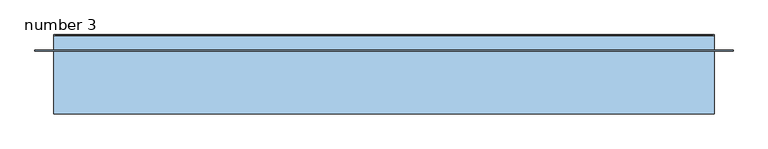
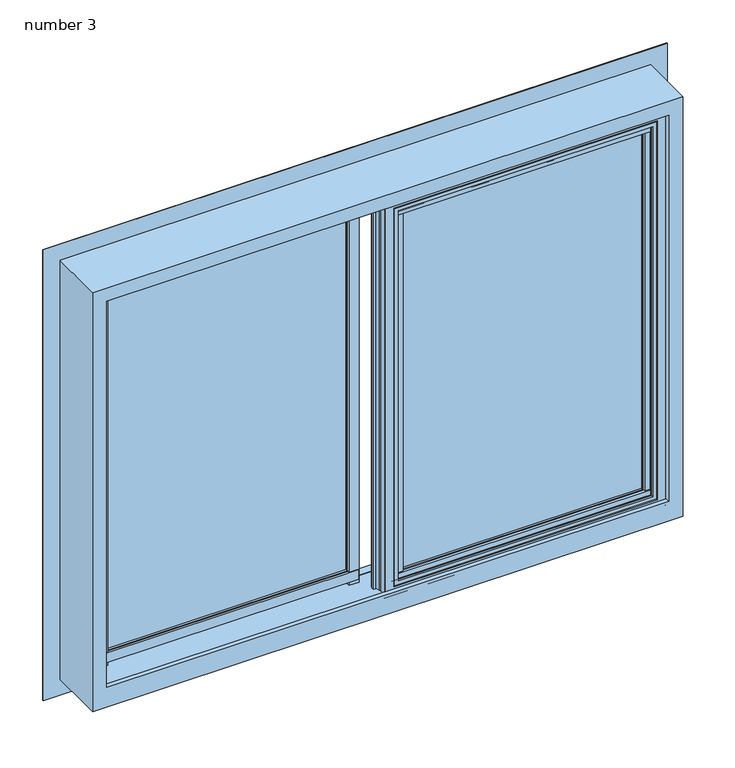
"""IFC4 building model written with IfcOpenShell, lengths in millimetres: window geometry, Window-Exterior-Sierra-Horizontal_Sliding_XO-36inch_Width-Standard : number 3."""

from ifc_helpers import new_model, si_unit, point, frame, frame_2d, origin, place, context, project, spatial, polyline, circle_curve, ellipse_curve, trimmed, segment, composite_curve, outline, extrude, faceted_brep, source, transform, mapped, element, save
from ifc_brep_helpers import plane_surface, cylinder_surface, revolved_surface, advanced_brep


def number_3_fed4ddc9(model_context):
    return source(origin(), model_context, "Body", "SolidModel", [
        extrude(outline(polyline([(-30.95625, 959.3990662), (-42.06875, 960.3157287), (-42.06875, 980.7896808), (-30.95625, 981.7063433), (-30.95625, 959.3990662)])), frame((23.8125, 0.0, 0.0), z_axis=(1.0, 0.0, 0.0), x_axis=(0.0, 1.0, 0.0)), (0.0, 0.0, 1.0), 536.575),
        extrude(outline(polyline([(-11.90625, 981.7063433), (-0.6945312, 980.9337774), (-0.6945312, 960.1716321), (-11.90625, 959.3990662), (-11.90625, 981.7063433)])), frame((23.8125, 0.0, 0.0), z_axis=(1.0, 0.0, 0.0), x_axis=(0.0, 1.0, 0.0)), (0.0, 0.0, 1.0), 536.575),
        extrude(outline(composite_curve([segment(polyline([(-30.95625, 970.5465365), (-30.95625, 959.4453125), (-33.62325, 959.4453125), (-33.62325, 961.0201125)]), True, "CONTINUOUS"), segment(trimmed(circle_curve(frame_2d((-31.4860105, 966.253572)), 5.6530426), [point((-33.62325, 961.0201125))], [point((-37.12845, 966.5996458))], False, "CARTESIAN"), True, "CONTINUOUS"), segment(polyline([(-37.12845, 966.5996458), (-41.275, 966.5996458), (-41.275, 974.5159792), (-39.5097, 974.5159792)]), True, "CONTINUOUS"), segment(trimmed(circle_curve(frame_2d((-31.4860105, 974.862053)), 8.0311494), [point((-39.5097, 974.5159792))], [point((-37.5778298, 980.0955125))], False, "CARTESIAN"), True, "CONTINUOUS"), segment(polyline([(-37.5778298, 980.0955125), (-37.5778298, 981.6703125), (-30.95625, 981.6703125), (-30.95625, 970.5465365)]), True, "CONTINUOUS")], self_intersect=False)), frame((23.8125, 0.0, 0.0), z_axis=(1.0, 0.0, 0.0), x_axis=(0.0, 1.0, 0.0)), (0.0, 0.0, 1.0), 536.575),
        extrude(outline(polyline([(13.890625, 959.3990662), (2.778125, 960.3157287), (2.778125, 980.7896808), (13.890625, 981.7063433), (13.890625, 959.3990662)])), frame((-560.3875, 0.0, 0.0), z_axis=(1.0, 0.0, 0.0), x_axis=(0.0, 1.0, 0.0)), (0.0, 0.0, 1.0), 536.575),
        extrude(outline(polyline([(32.940625, 981.7063433), (44.1523438, 980.9337774), (44.1523438, 960.1716321), (32.940625, 959.3990662), (32.940625, 981.7063433)])), frame((-560.3875, 0.0, 0.0), z_axis=(1.0, 0.0, 0.0), x_axis=(0.0, 1.0, 0.0)), (0.0, 0.0, 1.0), 536.575),
        extrude(outline(composite_curve([segment(polyline([(13.890625, 970.5465365), (13.890625, 959.4453125), (11.223625, 959.4453125), (11.223625, 961.0201125)]), True, "CONTINUOUS"), segment(trimmed(circle_curve(frame_2d((13.3608645, 966.253572)), 5.6530426), [point((11.223625, 961.0201125))], [point((7.718425, 966.5996458))], False, "CARTESIAN"), True, "CONTINUOUS"), segment(polyline([(7.718425, 966.5996458), (3.571875, 966.5996458), (3.571875, 974.5159792), (5.337175, 974.5159792)]), True, "CONTINUOUS"), segment(trimmed(circle_curve(frame_2d((13.3608645, 974.862053)), 8.0311494), [point((5.337175, 974.5159792))], [point((7.2690452, 980.0955125))], False, "CARTESIAN"), True, "CONTINUOUS"), segment(polyline([(7.2690452, 980.0955125), (7.2690452, 981.6703125), (13.890625, 981.6703125), (13.890625, 970.5465365)]), True, "CONTINUOUS")], self_intersect=False)), frame((-560.3875, 0.0, 0.0), z_axis=(1.0, 0.0, 0.0), x_axis=(0.0, 1.0, 0.0)), (0.0, 0.0, 1.0), 536.575),
        extrude(outline(polyline([(13.890625, 1761.4834412), (2.778125, 1762.4001037), (2.778125, 1782.8740558), (13.890625, 1783.7907183), (13.890625, 1761.4834412)])), frame((-560.3875, 0.0, 0.0), z_axis=(1.0, 0.0, 0.0), x_axis=(0.0, 1.0, 0.0)), (0.0, 0.0, 1.0), 536.575),
        extrude(outline(polyline([(32.940625, 1783.7907183), (44.1523438, 1783.0181524), (44.1523438, 1762.2560071), (32.940625, 1761.4834412), (32.940625, 1783.7907183)])), frame((-560.3875, 0.0, 0.0), z_axis=(1.0, 0.0, 0.0), x_axis=(0.0, 1.0, 0.0)), (0.0, 0.0, 1.0), 536.575),
        extrude(outline(composite_curve([segment(polyline([(13.890625, 1772.6309115), (13.890625, 1761.5296875), (11.223625, 1761.5296875), (11.223625, 1763.1044875)]), True, "CONTINUOUS"), segment(trimmed(circle_curve(frame_2d((13.3608645, 1768.337947)), 5.6530426), [point((11.223625, 1763.1044875))], [point((7.718425, 1768.6840208))], False, "CARTESIAN"), True, "CONTINUOUS"), segment(polyline([(7.718425, 1768.6840208), (3.571875, 1768.6840208), (3.571875, 1776.6003542), (5.337175, 1776.6003542)]), True, "CONTINUOUS"), segment(trimmed(circle_curve(frame_2d((13.3608645, 1776.946428)), 8.0311494), [point((5.337175, 1776.6003542))], [point((7.2690452, 1782.1798875))], False, "CARTESIAN"), True, "CONTINUOUS"), segment(polyline([(7.2690452, 1782.1798875), (7.2690452, 1783.7546875), (13.890625, 1783.7546875), (13.890625, 1772.6309115)]), True, "CONTINUOUS")], self_intersect=False)), frame((-560.3875, 0.0, 0.0), z_axis=(1.0, 0.0, 0.0), x_axis=(0.0, 1.0, 0.0)), (0.0, 0.0, 1.0), 536.575),
        extrude(outline(polyline([(-30.95625, 1761.4834412), (-42.06875, 1762.4001037), (-42.06875, 1782.8740558), (-30.95625, 1783.7907183), (-30.95625, 1761.4834412)])), frame((23.8125, 0.0, 0.0), z_axis=(1.0, 0.0, 0.0), x_axis=(0.0, 1.0, 0.0)), (0.0, 0.0, 1.0), 536.575),
        extrude(outline(polyline([(-11.90625, 1783.7907183), (-0.6945312, 1783.0181524), (-0.6945312, 1762.2560071), (-11.90625, 1761.4834412), (-11.90625, 1783.7907183)])), frame((23.8125, 0.0, 0.0), z_axis=(1.0, 0.0, 0.0), x_axis=(0.0, 1.0, 0.0)), (0.0, 0.0, 1.0), 536.575),
        extrude(outline(composite_curve([segment(polyline([(-30.95625, 1772.6309115), (-30.95625, 1761.5296875), (-33.62325, 1761.5296875), (-33.62325, 1763.1044875)]), True, "CONTINUOUS"), segment(trimmed(circle_curve(frame_2d((-31.4860105, 1768.337947)), 5.6530426), [point((-33.62325, 1763.1044875))], [point((-37.12845, 1768.6840208))], False, "CARTESIAN"), True, "CONTINUOUS"), segment(polyline([(-37.12845, 1768.6840208), (-41.275, 1768.6840208), (-41.275, 1776.6003542), (-39.5097, 1776.6003542)]), True, "CONTINUOUS"), segment(trimmed(circle_curve(frame_2d((-31.4860105, 1776.946428)), 8.0311494), [point((-39.5097, 1776.6003542))], [point((-37.5778298, 1782.1798875))], False, "CARTESIAN"), True, "CONTINUOUS"), segment(polyline([(-37.5778298, 1782.1798875), (-37.5778298, 1783.7546875), (-30.95625, 1783.7546875), (-30.95625, 1772.6309115)]), True, "CONTINUOUS")], self_intersect=False)), frame((23.8125, 0.0, 0.0), z_axis=(1.0, 0.0, 0.0), x_axis=(0.0, 1.0, 0.0)), (0.0, 0.0, 1.0), 536.575),
        extrude(outline(polyline([(-563.0134338, 13.890625), (-540.7061567, 13.890625), (-541.6228192, 4.365625), (-562.0967713, 4.365625), (-563.0134338, 13.890625)])), frame((0.0, 0.0, 952.5), z_axis=(0.0, 0.0, 1.0), x_axis=(1.0, 0.0, 0.0)), (0.0, 0.0, 1.0), 838.2),
        extrude(outline(polyline([(-540.7061567, 32.940625), (-563.0134338, 32.940625), (-562.2408679, 42.5648438), (-541.4787226, 42.5648438), (-540.7061567, 32.940625)])), frame((0.0, 0.0, 952.5), z_axis=(0.0, 0.0, 1.0), x_axis=(1.0, 0.0, 0.0)), (0.0, 0.0, 1.0), 838.2),
        extrude(outline(composite_curve([segment(polyline([(-551.8659635, 13.890625), (-540.7421875, 13.890625), (-540.7421875, 9.5985242), (-542.3169875, 9.5985242)]), True, "CONTINUOUS"), segment(trimmed(circle_curve(frame_2d((-547.550447, 13.3608645)), 6.445487), [point((-542.3169875, 9.5985242))], [point((-547.8965208, 6.924675))], False, "CARTESIAN"), True, "CONTINUOUS"), segment(polyline([(-547.8965208, 6.924675), (-547.8965208, 5.159375), (-555.8128542, 5.159375), (-555.8128542, 7.718425)]), True, "CONTINUOUS"), segment(trimmed(circle_curve(frame_2d((-556.158928, 13.3608645)), 5.6530426), [point((-555.8128542, 7.718425))], [point((-561.3923875, 11.223625))], False, "CARTESIAN"), True, "CONTINUOUS"), segment(polyline([(-561.3923875, 11.223625), (-562.9671875, 11.223625), (-562.9671875, 13.890625), (-551.8659635, 13.890625)]), True, "CONTINUOUS")], self_intersect=False)), frame((0.0, 0.0, 952.5), z_axis=(0.0, 0.0, 1.0), x_axis=(1.0, 0.0, 0.0)), (0.0, 0.0, 1.0), 838.2),
        extrude(outline(polyline([(563.0134338, -30.95625), (562.0967713, -40.48125), (541.6228192, -40.48125), (540.7061567, -30.95625), (563.0134338, -30.95625)])), frame((0.0, 0.0, 952.5), z_axis=(0.0, 0.0, 1.0), x_axis=(1.0, 0.0, 0.0)), (0.0, 0.0, 1.0), 838.2),
        extrude(outline(polyline([(540.7061567, -11.90625), (541.4787226, -2.2820312), (562.2408679, -2.2820312), (563.0134338, -11.90625), (540.7061567, -11.90625)])), frame((0.0, 0.0, 952.5), z_axis=(0.0, 0.0, 1.0), x_axis=(1.0, 0.0, 0.0)), (0.0, 0.0, 1.0), 838.2),
        extrude(outline(composite_curve([segment(polyline([(551.8659635, -30.95625), (562.9671875, -30.95625), (562.9671875, -33.62325), (561.3923875, -33.62325)]), True, "CONTINUOUS"), segment(trimmed(circle_curve(frame_2d((556.158928, -31.4860105)), 5.6530426), [point((561.3923875, -33.62325))], [point((555.8128542, -37.12845))], False, "CARTESIAN"), True, "CONTINUOUS"), segment(polyline([(555.8128542, -37.12845), (555.8128542, -39.6875), (547.8965208, -39.6875), (547.8965208, -37.9222)]), True, "CONTINUOUS"), segment(trimmed(circle_curve(frame_2d((547.550447, -31.4860105)), 6.445487), [point((547.8965208, -37.9222))], [point((542.3169875, -35.2483508))], False, "CARTESIAN"), True, "CONTINUOUS"), segment(polyline([(542.3169875, -35.2483508), (540.7421875, -35.2483508), (540.7421875, -30.95625), (551.8659635, -30.95625)]), True, "CONTINUOUS")], self_intersect=False)), frame((0.0, 0.0, 952.5), z_axis=(0.0, 0.0, 1.0), x_axis=(1.0, 0.0, 0.0)), (0.0, 0.0, 1.0), 838.2),
        extrude(outline(polyline([(879.8514818, 644.1495838), (1863.3495838, 644.1495838), (1863.3495838, -644.1495838), (879.8514818, -644.1495838), (879.8514818, 644.1495838)]), holes=[polyline([(914.4200683, -609.5809972), (1828.7809972, -609.5809972), (1828.7809972, 609.5809972), (914.4200683, 609.5809972), (914.4200683, -609.5809972)])]), frame((0.0, 56.35625, 0.0), z_axis=(0.0, 1.0, 0.0), x_axis=(0.0, 0.0, 1.0)), (0.0, 0.0, 1.0), 1.3692925),
        faceted_brep([(592.2452673, 61.8007595, 1811.4452673), (594.5632068, 85.439324, 1813.7632068), (594.5632068, 85.439324, 915.510409), (592.2452673, 61.8007595, 915.510409), (-592.2452673, 61.8007595, 1811.4452673), (-594.5632068, 85.439324, 1813.7632068), (-609.6, -59.8487004, 1828.8), (609.6, -59.8487004, 1828.8), (609.6, 83.8857584, 1828.8), (-609.6, 83.8857584, 1828.8), (-592.2452673, 61.8007595, 915.510409), (-594.5632068, 85.439324, 915.510409), (580.1297286, -59.8487004, 1799.3297286), (580.1297286, -48.9537259, 1799.3297286), (580.1297286, -48.9537259, 950.6555073), (580.1297286, -50.9012589, 951.1326574), (580.1297286, -50.9012589, 957.3267373), (580.1297286, -59.8487004, 957.3267373), (592.6836, -48.9537259, 1811.8836), (592.6836, -1.4525069, 1811.8836), (592.6836, -1.4525069, 939.0175967), (592.6836, -48.9537259, 950.6555073), (583.5400777, -1.4525069, 1802.7400777), (583.5400777, 10.1171482, 1802.7400777), (583.5400777, 10.1171482, 936.1830039), (583.5400777, -1.4525069, 939.0175967), (578.4551976, 10.1171482, 1797.6551976), (578.4551976, 26.899095, 1797.6551976), (578.4551976, 26.899095, 932.0713873), (578.4551976, 10.1171482, 936.1830039), (-609.6, 83.8857584, 915.510409), (-609.6, 86.3576576, 915.510409), (-609.6, 86.3576576, 914.4), (-609.6, -59.8487004, 914.4), (609.6, -59.8487004, 914.4), (609.6, 86.3576576, 914.4), (609.6, 86.3576576, 915.510409), (609.6, 83.8857584, 915.510409), (-580.1297286, -59.8487004, 1799.3297286), (-580.1297286, -59.8487004, 957.3267373), (-580.1297286, -50.9012589, 957.3267373), (-580.1297286, -50.9012589, 951.1326574), (583.6170827, 26.899095, 932.0713873), (583.6170827, 39.894466, 928.8874908), (573.8057011, 41.2733658, 928.5496571), (573.2593437, 52.0255869, 925.9153376), (582.3829219, 52.0255869, 925.9153376), (582.3829219, 55.096925, 925.1628525), (577.977436, 55.096925, 925.1628525), (577.977436, 56.33085, 924.860538), (-577.977436, 56.3169605, 924.8639409), (-577.977436, 55.096925, 925.1628525), (-582.3829219, 55.096925, 925.1628525), (-582.3829219, 52.0255869, 925.9153376), (-573.2593437, 52.0255869, 925.9153376), (-573.8057011, 41.2733658, 928.5496571), (-583.6170827, 39.894466, 928.8874908), (-583.6170827, 26.899095, 932.0713873), (-578.4551976, 26.899095, 932.0713873), (-578.4551976, 10.1171482, 936.1830039), (-583.5400777, 10.1171482, 936.1830039), (-583.5400777, -1.4525069, 939.0175967), (-592.6836, -1.4525069, 939.0175967), (-592.6836, -48.9537259, 950.6555073), (-580.1297286, -48.9537259, 950.6555073), (577.977436, 57.6604904, 924.8639409), (-577.977436, 57.6604904, 924.8639409), (577.977436, 57.6604904, 915.510409), (-577.977436, 57.6604904, 915.510409), (-580.1297286, -48.9537259, 1799.3297286), (-592.6836, -48.9537259, 1811.8836), (-592.6836, -1.4525069, 1811.8836), (-583.5400777, -1.4525069, 1802.7400777), (-583.5400777, 10.1171482, 1802.7400777), (-578.4551976, 10.1171482, 1797.6551976), (-578.4551976, 26.899095, 1797.6551976), (-583.6170827, 26.899095, 1802.8170827), (583.6170827, 26.899095, 1802.8170827), (583.6170827, 39.894466, 1802.8170827), (573.8057011, 41.2733658, 1793.0057011), (-583.6170827, 39.894466, 1802.8170827), (-605.917, 85.439324, 915.510409), (-605.917, 85.439324, 1825.117), (605.917, 85.439324, 1825.117), (605.917, 85.439324, 915.510409), (605.917, 77.5357584, 1825.117), (605.917, 77.5357584, 915.510409), (-605.917, 77.5357584, 1825.117), (-605.917, 77.5357584, 915.510409), (-608.203, 77.5357584, 915.510409), (-608.203, 77.5357584, 1827.403), (608.203, 77.5357584, 1827.403), (608.203, 77.5357584, 915.510409), (608.203, 83.8857584, 1827.403), (608.203, 83.8857584, 915.510409), (-608.203, 83.8857584, 1827.403), (-608.203, 83.8857584, 915.510409), (-584.2071742, 61.8007595, 915.510409), (-584.2071742, 60.6800805, 915.510409), (-577.977436, 60.6800805, 915.510409), (577.977436, 60.6800805, 915.510409), (584.2071742, 60.6800805, 915.510409), (584.2071742, 61.8007595, 915.510409), (-573.8057011, 41.2733658, 1793.0057011), (573.2593437, 52.0255869, 1792.4593437), (-573.2593437, 52.0255869, 1792.4593437), (-582.3829219, 52.0255869, 1801.5829219), (582.3829219, 52.0255869, 1801.5829219), (582.3829219, 55.096925, 1801.5829219), (-582.3829219, 55.096925, 1801.5829219), (-577.977436, 55.096925, 1797.177436), (577.977436, 55.096925, 1797.177436), (577.977436, 60.6800805, 1797.177436), (-577.977436, 60.6800805, 1797.177436), (-584.2071742, 60.6800805, 1803.4071742), (584.2071742, 60.6800805, 1803.4071742), (584.2071742, 61.8007595, 1803.4071742), (-584.2071742, 61.8007595, 1803.4071742)], [[[0, 1, 2, 3]], [[1, 0, 4, 5]], [[6, 7, 8, 9]], [[5, 4, 10, 11]], [[12, 13, 14, 15, 16, 17]], [[18, 19, 20, 21]], [[22, 23, 24, 25]], [[26, 27, 28, 29]], [[6, 9, 30, 31, 32, 33]], [[8, 7, 34, 35, 36, 37]], [[35, 34, 33, 32]], [[7, 6, 33, 34], [38, 12, 17, 39]], [[39, 17, 16, 40]], [[40, 16, 15, 41]], [[41, 15, 14, 21, 20, 25, 24, 29, 28, 42, 43, 44, 45, 46, 47, 48, 49, 50, 51, 52, 53, 54, 55, 56, 57, 58, 59, 60, 61, 62, 63, 64]], [[65, 66, 50, 49]], [[66, 65, 67, 68]], [[13, 69, 64, 63, 70, 18, 21, 14]], [[19, 71, 62, 61, 72, 22, 25, 20]], [[23, 73, 60, 59, 74, 26, 29, 24]], [[27, 75, 58, 57, 76, 77, 42, 28]], [[77, 78, 43, 42]], [[78, 79, 44, 43]], [[12, 38, 69, 13]], [[18, 70, 71, 19]], [[22, 72, 73, 23]], [[26, 74, 75, 27]], [[77, 76, 80, 78]], [[69, 38, 39, 40, 41, 64]], [[71, 70, 63, 62]], [[73, 72, 61, 60]], [[75, 74, 59, 58]], [[80, 76, 57, 56]], [[1, 5, 11, 81, 82, 83, 84, 2]], [[83, 85, 86, 84]], [[85, 87, 88, 89, 90, 91, 92, 86]], [[91, 93, 94, 92]], [[9, 8, 37, 94, 93, 95, 96, 30]], [[83, 82, 87, 85]], [[91, 90, 95, 93]], [[87, 82, 81, 88]], [[95, 90, 89, 96]], [[36, 31, 30, 96, 89, 88, 81, 11, 10, 97, 98, 99, 68, 67, 100, 101, 102, 3, 2, 84, 86, 92, 94, 37]], [[32, 31, 36, 35]], [[79, 78, 80, 103]], [[103, 80, 56, 55]], [[79, 104, 45, 44]], [[104, 105, 54, 53, 106, 107, 46, 45]], [[107, 108, 47, 46]], [[108, 109, 52, 51, 110, 111, 48, 47]], [[111, 112, 100, 67, 65, 49, 48]], [[112, 113, 99, 98, 114, 115, 101, 100]], [[115, 116, 102, 101]], [[4, 0, 3, 102, 116, 117, 97, 10]], [[79, 103, 105, 104]], [[107, 106, 109, 108]], [[111, 110, 113, 112]], [[115, 114, 117, 116]], [[105, 103, 55, 54]], [[109, 106, 53, 52]], [[113, 110, 51, 50, 66, 68, 99]], [[117, 114, 98, 97]]]),
        extrude(outline(polyline([(43.5040588, -30.95625), (42.5873963, -40.48125), (22.1134442, -40.48125), (21.1967817, -30.95625), (43.5040588, -30.95625)])), frame((0.0, 0.0, 952.5), z_axis=(0.0, 0.0, 1.0), x_axis=(1.0, 0.0, 0.0)), (0.0, 0.0, 1.0), 838.2),
        extrude(outline(polyline([(21.1967817, -11.90625), (21.9693476, -2.2820312), (42.7314929, -2.2820312), (43.5040588, -11.90625), (21.1967817, -11.90625)])), frame((0.0, 0.0, 952.5), z_axis=(0.0, 0.0, 1.0), x_axis=(1.0, 0.0, 0.0)), (0.0, 0.0, 1.0), 838.2),
        extrude(outline(composite_curve([segment(polyline([(32.3565885, -30.95625), (43.4578125, -30.95625), (43.4578125, -33.62325), (41.8830125, -33.62325)]), True, "CONTINUOUS"), segment(trimmed(circle_curve(frame_2d((36.649553, -31.4860105)), 5.6530426), [point((41.8830125, -33.62325))], [point((36.3034792, -37.12845))], False, "CARTESIAN"), True, "CONTINUOUS"), segment(polyline([(36.3034792, -37.12845), (36.3034792, -39.6875), (28.3871458, -39.6875), (28.3871458, -37.9222)]), True, "CONTINUOUS"), segment(trimmed(circle_curve(frame_2d((28.041072, -31.4860105)), 6.445487), [point((28.3871458, -37.9222))], [point((22.8076125, -35.2483508))], False, "CARTESIAN"), True, "CONTINUOUS"), segment(polyline([(22.8076125, -35.2483508), (21.2328125, -35.2483508), (21.2328125, -30.95625), (32.3565885, -30.95625)]), True, "CONTINUOUS")], self_intersect=False)), frame((0.0, 0.0, 952.5), z_axis=(0.0, 0.0, 1.0), x_axis=(1.0, 0.0, 0.0)), (0.0, 0.0, 1.0), 838.2),
        extrude(outline(polyline([(-43.5040588, 13.890625), (-21.1967817, 13.890625), (-22.1134442, 4.365625), (-42.5873963, 4.365625), (-43.5040588, 13.890625)])), frame((0.0, 0.0, 952.5), z_axis=(0.0, 0.0, 1.0), x_axis=(1.0, 0.0, 0.0)), (0.0, 0.0, 1.0), 838.2),
        extrude(outline(polyline([(-21.1967817, 32.940625), (-43.5040588, 32.940625), (-42.7314929, 42.5648438), (-21.9693476, 42.5648438), (-21.1967817, 32.940625)])), frame((0.0, 0.0, 952.5), z_axis=(0.0, 0.0, 1.0), x_axis=(1.0, 0.0, 0.0)), (0.0, 0.0, 1.0), 838.2),
        extrude(outline(composite_curve([segment(polyline([(-32.3565885, 13.890625), (-21.2328125, 13.890625), (-21.2328125, 9.5985242), (-22.8076125, 9.5985242)]), True, "CONTINUOUS"), segment(trimmed(circle_curve(frame_2d((-28.041072, 13.3608645)), 6.445487), [point((-22.8076125, 9.5985242))], [point((-28.3871458, 6.924675))], False, "CARTESIAN"), True, "CONTINUOUS"), segment(polyline([(-28.3871458, 6.924675), (-28.3871458, 5.159375), (-36.3034792, 5.159375), (-36.3034792, 7.718425)]), True, "CONTINUOUS"), segment(trimmed(circle_curve(frame_2d((-36.649553, 13.3608645)), 5.6530426), [point((-36.3034792, 7.718425))], [point((-41.8830125, 11.223625))], False, "CARTESIAN"), True, "CONTINUOUS"), segment(polyline([(-41.8830125, 11.223625), (-43.4578125, 11.223625), (-43.4578125, 13.890625), (-32.3565885, 13.890625)]), True, "CONTINUOUS")], self_intersect=False)), frame((0.0, 0.0, 952.5), z_axis=(0.0, 0.0, 1.0), x_axis=(1.0, 0.0, 0.0)), (0.0, 0.0, 1.0), 838.2),
        extrude(outline(polyline([(563.75935, -11.90625), (563.75935, -30.955332), (20.44065, -30.955332), (20.44065, -11.90625), (563.75935, -11.90625)])), frame((0.0, 0.0, 958.65315), z_axis=(0.0, 0.0, 1.0), x_axis=(1.0, 0.0, 0.0)), (0.0, 0.0, 1.0), 825.8937),
        advanced_brep(
        [(554.92015, -9.74725, 967.49235), (29.27985, -9.74725, 967.49235), (29.27985, -10.8831079, 967.49235), (554.92015, -10.8831079, 967.49235), (553.0833265, -7.3042106, 969.3291735), (31.1166735, -7.3042106, 969.3291735), (31.3062238, -9.74725, 969.5187238), (552.8937762, -9.74725, 969.5187238), (560.88915, -4.76885, 961.52335), (23.31085, -4.76885, 961.52335), (560.88915, -2.38125, 961.52335), (23.31085, -2.38125, 961.52335), (585.57795, -4.76885, 936.83455), (-1.37795, -4.76885, 936.83455), (1.00965, -2.38125, 939.22215), (583.19035, -2.38125, 939.22215), (585.57795, -7.33425, 936.83455), (-1.37795, -7.33425, 936.83455), (583.54595, -9.01065, 938.86655), (0.65405, -9.01065, 938.86655), (0.65405, -7.33425, 938.86655), (583.54595, -7.33425, 938.86655), (580.24395, -10.91565, 942.16855), (3.95605, -10.91565, 942.16855), (3.95605, -9.01065, 942.16855), (580.24395, -9.01065, 942.16855), (588.16875, -16.52905, 934.24375), (-3.96875, -16.52905, 934.24375), (-3.96875, -10.91565, 934.24375), (588.16875, -10.91565, 934.24375), (582.86015, -28.72105, 939.55235), (1.33985, -28.72105, 939.55235), (1.33985, -16.52905, 939.55235), (582.86015, -16.52905, 939.55235), (582.86015, -32.68345, 939.55235), (1.33985, -32.68345, 939.55235), (582.86015, -46.01845, 939.55235), (1.33985, -46.01845, 939.55235), (582.04735, -46.83125, 940.36515), (2.15265, -46.83125, 940.36515), (563.75935, -44.950732, 958.65315), (20.44065, -44.950732, 958.65315), (20.44065, -46.83125, 958.65315), (563.75935, -46.83125, 958.65315), (562.1584612, -46.550932, 960.2540388), (22.0415388, -46.550932, 960.2540388), (22.0415388, -44.950732, 960.2540388), (562.1584612, -44.950732, 960.2540388), (554.6146612, -42.7830125, 967.7978388), (29.5853388, -42.7830125, 967.7978388), (29.5853388, -46.550932, 967.7978388), (554.6146612, -46.550932, 967.7978388), (551.4396612, -30.955332, 970.9728388), (32.7603388, -30.955332, 970.9728388), (31.7476888, -42.7830125, 969.9601888), (552.4523112, -42.7830125, 969.9601888), (563.75935, -33.3436209, 958.65315), (20.44065, -33.3436209, 958.65315), (22.8289388, -30.955332, 961.0414388), (561.3710612, -30.955332, 961.0414388), (563.75935, -11.90625, 958.65315), (20.44065, -11.90625, 958.65315), (559.1555891, -10.8831079, 963.2569109), (25.0444109, -10.8831079, 963.2569109), (24.0212688, -11.90625, 962.2337688), (560.1787312, -11.90625, 962.2337688), (29.27985, -9.74725, 1775.70765), (29.27985, -10.8831079, 1775.70765), (31.1166735, -7.3042106, 1773.8708265), (31.3062238, -9.74725, 1773.6812762), (23.31085, -4.76885, 1781.67665), (23.31085, -2.38125, 1781.67665), (-1.37795, -4.76885, 1806.36545), (1.00965, -2.38125, 1803.97785), (-1.37795, -7.33425, 1806.36545), (0.65405, -9.01065, 1804.33345), (0.65405, -7.33425, 1804.33345), (3.95605, -10.91565, 1801.03145), (3.95605, -9.01065, 1801.03145), (-3.96875, -16.52905, 1808.95625), (-3.96875, -10.91565, 1808.95625), (1.33985, -28.72105, 1803.64765), (1.33985, -16.52905, 1803.64765), (1.33985, -32.68345, 1803.64765), (1.33985, -46.01845, 1803.64765), (2.15265, -46.83125, 1802.83485), (20.44065, -44.950732, 1784.54685), (20.44065, -46.83125, 1784.54685), (22.0415388, -46.550932, 1782.9459612), (22.0415388, -44.950732, 1782.9459612), (29.5853388, -42.7830125, 1775.4021612), (29.5853388, -46.550932, 1775.4021612), (32.7603388, -30.955332, 1772.2271612), (31.7476888, -42.7830125, 1773.2398112), (20.44065, -33.3436209, 1784.54685), (22.8289388, -30.955332, 1782.1585612), (20.44065, -11.90625, 1784.54685), (25.0444109, -10.8831079, 1779.9430891), (24.0212688, -11.90625, 1780.9662312), (554.92015, -9.74725, 1775.70765), (554.92015, -10.8831079, 1775.70765), (553.0833265, -7.3042106, 1773.8708265), (552.8937762, -9.74725, 1773.6812762), (560.88915, -4.76885, 1781.67665), (560.88915, -2.38125, 1781.67665), (585.57795, -4.76885, 1806.36545), (583.19035, -2.38125, 1803.97785), (585.57795, -7.33425, 1806.36545), (583.54595, -9.01065, 1804.33345), (583.54595, -7.33425, 1804.33345), (580.24395, -10.91565, 1801.03145), (580.24395, -9.01065, 1801.03145), (588.16875, -16.52905, 1808.95625), (588.16875, -10.91565, 1808.95625), (582.86015, -28.72105, 1803.64765), (582.86015, -16.52905, 1803.64765), (582.86015, -32.68345, 1803.64765), (582.86015, -46.01845, 1803.64765), (582.04735, -46.83125, 1802.83485), (563.75935, -44.950732, 1784.54685), (563.75935, -46.83125, 1784.54685), (562.1584612, -46.550932, 1782.9459612), (562.1584612, -44.950732, 1782.9459612), (554.6146612, -42.7830125, 1775.4021612), (554.6146612, -46.550932, 1775.4021612), (551.4396612, -30.955332, 1772.2271612), (552.4523112, -42.7830125, 1773.2398112), (563.75935, -33.3436209, 1784.54685), (561.3710612, -30.955332, 1782.1585612), (563.75935, -11.90625, 1784.54685), (559.1555891, -10.8831079, 1779.9430891), (560.1787312, -11.90625, 1780.9662312)],
        [
            (0, 1),
            (1, 2),
            (2, 3),
            (3, 0),
            (4, 5),
            (5, 6),
            (6, 7),
            (7, 4),
            (8, 9),
            (9, 5),
            (4, 8),
            (10, 11),
            (11, 9),
            (8, 10),
            (12, 13),
            (13, 14, ellipse_curve(frame((1.00965, -4.76885, 939.22215), z_axis=(0.7071067811865475, 0.0, -0.7071067811865475), x_axis=(0.7071067811865476, 0.0, 0.7071067811865474)), 3.3765763, 2.3876)),
            (14, 15),
            (15, 12, ellipse_curve(frame((583.19035, -4.76885, 939.22215), z_axis=(-0.7071067811865475, 0.0, -0.7071067811865475), x_axis=(0.7071067811865476, 0.0, -0.7071067811865474)), 3.3765763, 2.3876)),
            (16, 17),
            (17, 13),
            (12, 16),
            (18, 19),
            (19, 20),
            (20, 21),
            (21, 18),
            (22, 23),
            (23, 24),
            (24, 25),
            (25, 22),
            (26, 27),
            (27, 28),
            (28, 29),
            (29, 26),
            (30, 31),
            (31, 32),
            (32, 33),
            (33, 30),
            (34, 35),
            (35, 31, ellipse_curve(frame((1.33985, -30.70225, 939.55235), z_axis=(-0.7071067811865475, 0.0, 0.7071067811865475), x_axis=(-0.7071067811865476, 0.0, -0.7071067811865474)), 2.8018399, 1.9812)),
            (30, 34, ellipse_curve(frame((582.86015, -30.70225, 939.55235), z_axis=(0.7071067811865475, 0.0, 0.7071067811865475), x_axis=(-0.7071067811865476, 0.0, 0.7071067811865474)), 2.8018399, 1.9812)),
            (36, 37),
            (37, 35),
            (34, 36),
            (38, 39),
            (39, 37, ellipse_curve(frame((2.15265, -46.01845, 940.36515), z_axis=(0.7071067811865475, 0.0, -0.7071067811865475), x_axis=(0.7071067811865476, 0.0, 0.7071067811865474)), 1.1494728, 0.8128)),
            (36, 38, ellipse_curve(frame((582.04735, -46.01845, 940.36515), z_axis=(-0.7071067811865475, 0.0, -0.7071067811865475), x_axis=(0.7071067811865476, 0.0, -0.7071067811865474)), 1.1494728, 0.8128)),
            (40, 41),
            (41, 42),
            (42, 43),
            (43, 40),
            (44, 45),
            (45, 46),
            (46, 47),
            (47, 44),
            (48, 49),
            (49, 50),
            (50, 51),
            (51, 48),
            (52, 53),
            (53, 54),
            (54, 55),
            (55, 52),
            (56, 57),
            (57, 58),
            (58, 59),
            (59, 56),
            (60, 61),
            (61, 57),
            (56, 60),
            (62, 63),
            (63, 64),
            (64, 65),
            (65, 62),
            (1, 66),
            (66, 67),
            (67, 2),
            (5, 68),
            (68, 69),
            (69, 6),
            (9, 70),
            (70, 68),
            (11, 71),
            (71, 70),
            (13, 72),
            (72, 73, ellipse_curve(frame((1.00965, -4.76885, 1803.97785), z_axis=(-0.7071067811865475, 0.0, -0.7071067811865475), x_axis=(0.7071067811865474, 0.0, -0.7071067811865476)), 3.3765763, 2.3876)),
            (73, 14),
            (17, 74),
            (74, 72),
            (19, 75),
            (75, 76),
            (76, 20),
            (23, 77),
            (77, 78),
            (78, 24),
            (27, 79),
            (79, 80),
            (80, 28),
            (31, 81),
            (81, 82),
            (82, 32),
            (35, 83),
            (83, 81, ellipse_curve(frame((1.33985, -30.70225, 1803.64765), z_axis=(0.7071067811865475, 0.0, 0.7071067811865475), x_axis=(-0.7071067811865474, 0.0, 0.7071067811865476)), 2.8018399, 1.9812)),
            (37, 84),
            (84, 83),
            (39, 85),
            (85, 84, ellipse_curve(frame((2.15265, -46.01845, 1802.83485), z_axis=(-0.7071067811865475, 0.0, -0.7071067811865475), x_axis=(0.7071067811865474, 0.0, -0.7071067811865476)), 1.1494728, 0.8128)),
            (41, 86),
            (86, 87),
            (87, 42),
            (45, 88),
            (88, 89),
            (89, 46),
            (49, 90),
            (90, 91),
            (91, 50),
            (53, 92),
            (92, 93),
            (93, 54),
            (57, 94),
            (94, 95),
            (95, 58),
            (61, 96),
            (96, 94),
            (63, 97),
            (97, 98),
            (98, 64),
            (66, 99),
            (99, 100),
            (100, 67),
            (68, 101),
            (101, 102),
            (102, 69),
            (70, 103),
            (103, 101),
            (71, 104),
            (104, 103),
            (72, 105),
            (105, 106, ellipse_curve(frame((583.19035, -4.76885, 1803.97785), z_axis=(-0.7071067811865475, 0.0, 0.7071067811865475), x_axis=(-0.7071067811865476, 0.0, -0.7071067811865474)), 3.3765763, 2.3876)),
            (106, 73),
            (74, 107),
            (107, 105),
            (75, 108),
            (108, 109),
            (109, 76),
            (77, 110),
            (110, 111),
            (111, 78),
            (79, 112),
            (112, 113),
            (113, 80),
            (81, 114),
            (114, 115),
            (115, 82),
            (83, 116),
            (116, 114, ellipse_curve(frame((582.86015, -30.70225, 1803.64765), z_axis=(0.7071067811865475, 0.0, -0.7071067811865475), x_axis=(0.7071067811865476, 0.0, 0.7071067811865474)), 2.8018399, 1.9812)),
            (84, 117),
            (117, 116),
            (85, 118),
            (118, 117, ellipse_curve(frame((582.04735, -46.01845, 1802.83485), z_axis=(-0.7071067811865475, 0.0, 0.7071067811865475), x_axis=(-0.7071067811865476, 0.0, -0.7071067811865474)), 1.1494728, 0.8128)),
            (86, 119),
            (119, 120),
            (120, 87),
            (88, 121),
            (121, 122),
            (122, 89),
            (90, 123),
            (123, 124),
            (124, 91),
            (92, 125),
            (125, 126),
            (126, 93),
            (94, 127),
            (127, 128),
            (128, 95),
            (96, 129),
            (129, 127),
            (97, 130),
            (130, 131),
            (131, 98),
            (62, 130),
            (100, 3),
            (99, 0),
            (102, 7),
            (101, 4),
            (103, 8),
            (104, 10),
            (106, 15),
            (105, 12),
            (107, 16),
            (109, 21),
            (108, 18),
            (111, 25),
            (110, 22),
            (113, 29),
            (112, 26),
            (115, 33),
            (114, 30),
            (116, 34),
            (117, 36),
            (118, 38),
            (120, 43),
            (119, 40),
            (122, 47),
            (121, 44),
            (124, 51),
            (123, 48),
            (126, 55),
            (125, 52),
            (128, 59),
            (127, 56),
            (129, 60),
            (131, 65),
        ],
        [
            plane_surface(frame((554.92015, -10.8831079, 967.49235), z_axis=(0.0, 0.0, 1.0), x_axis=(-1.0, 0.0, 0.0))),
            plane_surface(frame((552.8937762, -9.74725, 969.5187238), z_axis=(0.0, 0.07735544009934271, 0.9970035786731345), x_axis=(-1.0, 0.0, 0.0))),
            plane_surface(frame((553.0833265, -7.3042106, 969.3291735), z_axis=(0.0, 0.9510889261909004, 0.3089172291683326), x_axis=(-1.0, 0.0, 0.0))),
            plane_surface(frame((560.88915, -4.76885, 961.52335), z_axis=(0.0, 0.0, 1.0), x_axis=(-1.0, 0.0, 0.0))),
            cylinder_surface(frame((588.16875, -4.76885, 939.22215), z_axis=(1.0, 0.0, 0.0), x_axis=(0.0, -1.0, 0.0)), 2.3876),
            plane_surface(frame((585.57795, -4.76885, 936.83455), z_axis=(0.0, 0.0, -1.0), x_axis=(-1.0, 0.0, 0.0))),
            plane_surface(frame((583.54595, -7.33425, 938.86655), z_axis=(0.0, 0.0, -1.0), x_axis=(-1.0, 0.0, 0.0))),
            plane_surface(frame((580.24395, -9.01065, 942.16855), z_axis=(0.0, 0.0, -1.0), x_axis=(-1.0, 0.0, 0.0))),
            plane_surface(frame((588.16875, -10.91565, 934.24375), z_axis=(0.0, 0.0, -1.0), x_axis=(-1.0, 0.0, 0.0))),
            plane_surface(frame((582.86015, -16.52905, 939.55235), z_axis=(0.0, 0.0, -1.0), x_axis=(-1.0, 0.0, 0.0))),
            revolved_surface(polyline([(-0.6413499930890794, -32.68345, 939.55235), (584.841349993089, -32.68345, 939.55235)]), (588.16875, -30.70225, 939.55235), (-1.0, 0.0, 0.0)),
            plane_surface(frame((582.86015, -32.68345, 939.55235), z_axis=(0.0, 0.0, -1.0), x_axis=(-1.0, 0.0, 0.0))),
            cylinder_surface(frame((588.16875, -46.01845, 940.36515), z_axis=(1.0, 0.0, 0.0), x_axis=(0.0, -1.0, 0.0)), 0.8128),
            plane_surface(frame((563.75935, -46.83125, 958.65315), z_axis=(0.0, 0.0, 1.0), x_axis=(-1.0, 0.0, 0.0))),
            plane_surface(frame((562.1584612, -44.950732, 960.2540388), z_axis=(0.0, 0.0, -1.0), x_axis=(-1.0, 0.0, 0.0))),
            plane_surface(frame((554.6146612, -46.550932, 967.7978388), z_axis=(0.0, 0.0, 1.0), x_axis=(-1.0, 0.0, 0.0))),
            plane_surface(frame((552.4523112, -42.7830125, 969.9601888), z_axis=(0.0, -0.08530487454184647, 0.996354895797376), x_axis=(-1.0, 0.0, 0.0))),
            plane_surface(frame((561.3710612, -30.955332, 961.0414388), z_axis=(0.0, 0.7071067811865713, -0.7071067811865238), x_axis=(-1.0, 0.0, 0.0))),
            plane_surface(frame((563.75935, -33.3436209, 958.65315), z_axis=(0.0, 0.0, 1.0), x_axis=(-1.0, 0.0, 0.0))),
            plane_surface(frame((560.1787312, -11.90625, 962.2337688), z_axis=(0.0, -0.7071067811861558, 0.7071067811869393), x_axis=(-1.0, 0.0, 0.0))),
            plane_surface(frame((29.27985, -10.8831079, 967.49235), z_axis=(1.0, 0.0, 0.0), x_axis=(0.0, 0.0, 1.0))),
            plane_surface(frame((31.3062238, -9.74725, 969.5187238), z_axis=(0.9970035786731345, 0.07735544009934266, 0.0), x_axis=(0.0, 0.0, 1.0))),
            plane_surface(frame((31.1166735, -7.3042106, 969.3291735), z_axis=(0.30891722916833264, 0.9510889261909004, 0.0), x_axis=(0.0, 0.0, 1.0))),
            plane_surface(frame((23.31085, -4.76885, 961.52335), z_axis=(1.0, 0.0, 0.0), x_axis=(0.0, 0.0, 1.0))),
            cylinder_surface(frame((1.00965, -4.76885, 934.24375), z_axis=(0.0, 0.0, -1.0), x_axis=(0.0, -1.0, 0.0)), 2.3876),
            plane_surface(frame((-1.37795, -4.76885, 936.83455), z_axis=(-1.0, 0.0, 0.0), x_axis=(0.0, 0.0, 1.0))),
            plane_surface(frame((0.65405, -7.33425, 938.86655), z_axis=(-1.0, 0.0, 0.0), x_axis=(0.0, 0.0, 1.0))),
            plane_surface(frame((3.95605, -9.01065, 942.16855), z_axis=(-1.0, 0.0, 0.0), x_axis=(0.0, 0.0, 1.0))),
            plane_surface(frame((-3.96875, -10.91565, 934.24375), z_axis=(-1.0, 0.0, 0.0), x_axis=(0.0, 0.0, 1.0))),
            plane_surface(frame((1.33985, -16.52905, 939.55235), z_axis=(-1.0, 0.0, 0.0), x_axis=(0.0, 0.0, 1.0))),
            revolved_surface(polyline([(1.33985, -32.68345, 1805.6288499930893), (1.33985, -32.68345, 937.571150006911)]), (1.33985, -30.70225, 934.24375), (0.0, 0.0, 1.0)),
            plane_surface(frame((1.33985, -32.68345, 939.55235), z_axis=(-1.0, 0.0, 0.0), x_axis=(0.0, 0.0, 1.0))),
            cylinder_surface(frame((2.15265, -46.01845, 934.24375), z_axis=(0.0, 0.0, -1.0), x_axis=(0.0, -1.0, 0.0)), 0.8128),
            plane_surface(frame((20.44065, -46.83125, 958.65315), z_axis=(1.0, 0.0, 0.0), x_axis=(0.0, 0.0, 1.0))),
            plane_surface(frame((22.0415388, -44.950732, 960.2540388), z_axis=(-1.0, 0.0, 0.0), x_axis=(0.0, 0.0, 1.0))),
            plane_surface(frame((29.5853388, -46.550932, 967.7978388), z_axis=(1.0, 0.0, 0.0), x_axis=(0.0, 0.0, 1.0))),
            plane_surface(frame((31.7476888, -42.7830125, 969.9601888), z_axis=(0.996354895797376, -0.08530487454184653, 0.0), x_axis=(0.0, 0.0, 1.0))),
            plane_surface(frame((22.8289388, -30.955332, 961.0414388), z_axis=(-0.7071067811865238, 0.7071067811865713, 0.0), x_axis=(0.0, 0.0, 1.0))),
            plane_surface(frame((20.44065, -33.3436209, 958.65315), z_axis=(1.0, 0.0, 0.0), x_axis=(0.0, 0.0, 1.0))),
            plane_surface(frame((24.0212688, -11.90625, 962.2337688), z_axis=(0.7071067811869393, -0.7071067811861558, 0.0), x_axis=(0.0, 0.0, 1.0))),
            plane_surface(frame((29.27985, -10.8831079, 1775.70765), z_axis=(0.0, 0.0, -1.0), x_axis=(1.0, 0.0, 0.0))),
            plane_surface(frame((31.3062238, -9.74725, 1773.6812762), z_axis=(0.0, 0.0773554400993426, -0.9970035786731345), x_axis=(1.0, 0.0, 0.0))),
            plane_surface(frame((31.1166735, -7.3042106, 1773.8708265), z_axis=(0.0, 0.9510889261909004, -0.3089172291683327), x_axis=(1.0, 0.0, 0.0))),
            plane_surface(frame((23.31085, -4.76885, 1781.67665), z_axis=(0.0, 0.0, -1.0), x_axis=(1.0, 0.0, 0.0))),
            cylinder_surface(frame((-3.96875, -4.76885, 1803.97785), z_axis=(-1.0, 0.0, 0.0), x_axis=(0.0, -1.0, 0.0)), 2.3876),
            plane_surface(frame((-1.37795, -4.76885, 1806.36545), z_axis=(0.0, 0.0, 1.0), x_axis=(1.0, 0.0, 0.0))),
            plane_surface(frame((0.65405, -7.33425, 1804.33345), z_axis=(0.0, 0.0, 1.0), x_axis=(1.0, 0.0, 0.0))),
            plane_surface(frame((3.95605, -9.01065, 1801.03145), z_axis=(0.0, 0.0, 1.0), x_axis=(1.0, 0.0, 0.0))),
            plane_surface(frame((-3.96875, -10.91565, 1808.95625), z_axis=(0.0, 0.0, 1.0), x_axis=(1.0, 0.0, 0.0))),
            plane_surface(frame((1.33985, -16.52905, 1803.64765), z_axis=(0.0, 0.0, 1.0), x_axis=(1.0, 0.0, 0.0))),
            revolved_surface(polyline([(584.841349993089, -32.68345, 1803.64765), (-0.6413499930890376, -32.68345, 1803.64765)]), (-3.96875, -30.70225, 1803.64765), (1.0, 0.0, 0.0)),
            plane_surface(frame((1.33985, -32.68345, 1803.64765), z_axis=(0.0, 0.0, 1.0), x_axis=(1.0, 0.0, 0.0))),
            cylinder_surface(frame((-3.96875, -46.01845, 1802.83485), z_axis=(-1.0, 0.0, 0.0), x_axis=(0.0, -1.0, 0.0)), 0.8128),
            plane_surface(frame((20.44065, -46.83125, 1784.54685), z_axis=(0.0, 0.0, -1.0), x_axis=(1.0, 0.0, 0.0))),
            plane_surface(frame((22.0415388, -44.950732, 1782.9459612), z_axis=(0.0, 0.0, 1.0), x_axis=(1.0, 0.0, 0.0))),
            plane_surface(frame((29.5853388, -46.550932, 1775.4021612), z_axis=(0.0, 0.0, -1.0), x_axis=(1.0, 0.0, 0.0))),
            plane_surface(frame((31.7476888, -42.7830125, 1773.2398112), z_axis=(0.0, -0.08530487454184658, -0.996354895797376), x_axis=(1.0, 0.0, 0.0))),
            plane_surface(frame((22.8289388, -30.955332, 1782.1585612), z_axis=(0.0, 0.7071067811865713, 0.7071067811865238), x_axis=(1.0, 0.0, 0.0))),
            plane_surface(frame((20.44065, -33.3436209, 1784.54685), z_axis=(0.0, 0.0, -1.0), x_axis=(1.0, 0.0, 0.0))),
            plane_surface(frame((24.0212688, -11.90625, 1780.9662312), z_axis=(0.0, -0.7071067811861558, -0.7071067811869393), x_axis=(1.0, 0.0, 0.0))),
            plane_surface(frame((559.1555891, -10.8831079, 1779.9430891), z_axis=(0.0, -1.0, 0.0), x_axis=(0.0, 0.0, -1.0))),
            plane_surface(frame((554.92015, -10.8831079, 1775.70765), z_axis=(-1.0, 0.0, 0.0), x_axis=(0.0, 0.0, -1.0))),
            plane_surface(frame((554.92015, -9.74725, 1775.70765), z_axis=(0.0, -1.0, 0.0), x_axis=(0.0, 0.0, -1.0))),
            plane_surface(frame((552.8937762, -9.74725, 1773.6812762), z_axis=(-0.9970035786731345, 0.07735544009934266, 0.0), x_axis=(0.0, 0.0, -1.0))),
            plane_surface(frame((553.0833265, -7.3042106, 1773.8708265), z_axis=(-0.30891722916833264, 0.9510889261909004, 0.0), x_axis=(0.0, 0.0, -1.0))),
            plane_surface(frame((560.88915, -4.76885, 1781.67665), z_axis=(-1.0, 0.0, 0.0), x_axis=(0.0, 0.0, -1.0))),
            plane_surface(frame((560.88915, -2.38125, 1781.67665), z_axis=(0.0, 1.0, 0.0), x_axis=(0.0, 0.0, -1.0))),
            cylinder_surface(frame((583.19035, -4.76885, 1808.95625), z_axis=(0.0, 0.0, 1.0), x_axis=(0.0, -1.0, 0.0)), 2.3876),
            plane_surface(frame((585.57795, -4.76885, 1806.36545), z_axis=(1.0, 0.0, 0.0), x_axis=(0.0, 0.0, -1.0))),
            plane_surface(frame((585.57795, -7.33425, 1806.36545), z_axis=(0.0, -1.0, 0.0), x_axis=(0.0, 0.0, -1.0))),
            plane_surface(frame((583.54595, -7.33425, 1804.33345), z_axis=(1.0, 0.0, 0.0), x_axis=(0.0, 0.0, -1.0))),
            plane_surface(frame((583.54595, -9.01065, 1804.33345), z_axis=(0.0, -1.0, 0.0), x_axis=(0.0, 0.0, -1.0))),
            plane_surface(frame((580.24395, -9.01065, 1801.03145), z_axis=(1.0, 0.0, 0.0), x_axis=(0.0, 0.0, -1.0))),
            plane_surface(frame((580.24395, -10.91565, 1801.03145), z_axis=(0.0, 1.0, 0.0), x_axis=(0.0, 0.0, -1.0))),
            plane_surface(frame((588.16875, -10.91565, 1808.95625), z_axis=(1.0, 0.0, 0.0), x_axis=(0.0, 0.0, -1.0))),
            plane_surface(frame((588.16875, -16.52905, 1808.95625), z_axis=(0.0, -1.0, 0.0), x_axis=(0.0, 0.0, -1.0))),
            plane_surface(frame((582.86015, -16.52905, 1803.64765), z_axis=(1.0, 0.0, 0.0), x_axis=(0.0, 0.0, -1.0))),
            revolved_surface(polyline([(582.86015, -32.68345, 937.571150006911), (582.86015, -32.68345, 1805.6288499930893)]), (582.86015, -30.70225, 1808.95625), (0.0, 0.0, -1.0)),
            plane_surface(frame((582.86015, -32.68345, 1803.64765), z_axis=(1.0, 0.0, 0.0), x_axis=(0.0, 0.0, -1.0))),
            cylinder_surface(frame((582.04735, -46.01845, 1808.95625), z_axis=(0.0, 0.0, 1.0), x_axis=(0.0, -1.0, 0.0)), 0.8128),
            plane_surface(frame((582.04735, -46.83125, 1802.83485), z_axis=(0.0, -1.0, 0.0), x_axis=(0.0, 0.0, -1.0))),
            plane_surface(frame((563.75935, -46.83125, 1784.54685), z_axis=(-1.0, 0.0, 0.0), x_axis=(0.0, 0.0, -1.0))),
            plane_surface(frame((563.75935, -44.950732, 1784.54685), z_axis=(0.0, -1.0, 0.0), x_axis=(0.0, 0.0, -1.0))),
            plane_surface(frame((562.1584612, -44.950732, 1782.9459612), z_axis=(1.0, 0.0, 0.0), x_axis=(0.0, 0.0, -1.0))),
            plane_surface(frame((562.1584612, -46.550932, 1782.9459612), z_axis=(0.0, -1.0, 0.0), x_axis=(0.0, 0.0, -1.0))),
            plane_surface(frame((554.6146612, -46.550932, 1775.4021612), z_axis=(-1.0, 0.0, 0.0), x_axis=(0.0, 0.0, -1.0))),
            plane_surface(frame((554.6146612, -42.7830125, 1775.4021612), z_axis=(0.0, -1.0, 0.0), x_axis=(0.0, 0.0, -1.0))),
            plane_surface(frame((552.4523112, -42.7830125, 1773.2398112), z_axis=(-0.996354895797376, -0.08530487454184653, 0.0), x_axis=(0.0, 0.0, -1.0))),
            plane_surface(frame((551.4396612, -30.955332, 1772.2271612), z_axis=(0.0, 1.0, 0.0), x_axis=(0.0, 0.0, -1.0))),
            plane_surface(frame((561.3710612, -30.955332, 1782.1585612), z_axis=(0.7071067811865238, 0.7071067811865713, 0.0), x_axis=(0.0, 0.0, -1.0))),
            plane_surface(frame((563.75935, -33.3436209, 1784.54685), z_axis=(-1.0, 0.0, 0.0), x_axis=(0.0, 0.0, -1.0))),
            plane_surface(frame((563.75935, -11.90625, 1784.54685), z_axis=(0.0, -1.0, 0.0), x_axis=(0.0, 0.0, -1.0))),
            plane_surface(frame((560.1787312, -11.90625, 1780.9662312), z_axis=(-0.7071067811869393, -0.7071067811861558, 0.0), x_axis=(0.0, 0.0, -1.0))),
        ],
        [
            (0, [[1, 2, 3, 4]]),
            (1, [[5, 6, 7, 8]]),
            (2, [[9, 10, -5, 11]]),
            (3, [[12, 13, -9, 14]]),
            (4, [[15, 16, 17, 18]]),
            (5, [[19, 20, -15, 21]]),
            (6, [[22, 23, 24, 25]]),
            (7, [[26, 27, 28, 29]]),
            (8, [[30, 31, 32, 33]]),
            (9, [[34, 35, 36, 37]]),
            (10, [[38, 39, -34, 40]]),
            (11, [[41, 42, -38, 43]]),
            (12, [[44, 45, -41, 46]]),
            (13, [[47, 48, 49, 50]]),
            (14, [[51, 52, 53, 54]]),
            (15, [[55, 56, 57, 58]]),
            (16, [[59, 60, 61, 62]]),
            (17, [[63, 64, 65, 66]]),
            (18, [[67, 68, -63, 69]]),
            (19, [[70, 71, 72, 73]]),
            (20, [[74, 75, 76, -2]]),
            (21, [[77, 78, 79, -6]]),
            (22, [[80, 81, -77, -10]]),
            (23, [[82, 83, -80, -13]]),
            (24, [[84, 85, 86, -16]]),
            (25, [[87, 88, -84, -20]]),
            (26, [[89, 90, 91, -23]]),
            (27, [[92, 93, 94, -27]]),
            (28, [[95, 96, 97, -31]]),
            (29, [[98, 99, 100, -35]]),
            (30, [[101, 102, -98, -39]]),
            (31, [[103, 104, -101, -42]]),
            (32, [[105, 106, -103, -45]]),
            (33, [[107, 108, 109, -48]]),
            (34, [[110, 111, 112, -52]]),
            (35, [[113, 114, 115, -56]]),
            (36, [[116, 117, 118, -60]]),
            (37, [[119, 120, 121, -64]]),
            (38, [[122, 123, -119, -68]]),
            (39, [[124, 125, 126, -71]]),
            (40, [[127, 128, 129, -75]]),
            (41, [[130, 131, 132, -78]]),
            (42, [[133, 134, -130, -81]]),
            (43, [[135, 136, -133, -83]]),
            (44, [[137, 138, 139, -85]]),
            (45, [[140, 141, -137, -88]]),
            (46, [[142, 143, 144, -90]]),
            (47, [[145, 146, 147, -93]]),
            (48, [[148, 149, 150, -96]]),
            (49, [[151, 152, 153, -99]]),
            (50, [[154, 155, -151, -102]]),
            (51, [[156, 157, -154, -104]]),
            (52, [[158, 159, -156, -106]]),
            (53, [[160, 161, 162, -108]]),
            (54, [[163, 164, 165, -111]]),
            (55, [[166, 167, 168, -114]]),
            (56, [[169, 170, 171, -117]]),
            (57, [[172, 173, 174, -120]]),
            (58, [[175, 176, -172, -123]]),
            (59, [[177, 178, 179, -125]]),
            (60, [[-70, 180, -177, -124], [-3, -76, -129, 181]]),
            (61, [[182, -4, -181, -128]]),
            (62, [[-1, -182, -127, -74], [-7, -79, -132, 183]]),
            (63, [[184, -8, -183, -131]]),
            (64, [[185, -11, -184, -134]]),
            (65, [[186, -14, -185, -136]]),
            (66, [[-17, -86, -139, 187], [-12, -186, -135, -82]]),
            (67, [[188, -18, -187, -138]]),
            (68, [[189, -21, -188, -141]]),
            (69, [[-19, -189, -140, -87], [-24, -91, -144, 190]]),
            (70, [[191, -25, -190, -143]]),
            (71, [[-22, -191, -142, -89], [-28, -94, -147, 192]]),
            (72, [[193, -29, -192, -146]]),
            (73, [[-32, -97, -150, 194], [-26, -193, -145, -92]]),
            (74, [[195, -33, -194, -149]]),
            (75, [[-30, -195, -148, -95], [-36, -100, -153, 196]]),
            (76, [[197, -37, -196, -152]]),
            (77, [[198, -40, -197, -155]]),
            (78, [[199, -43, -198, -157]]),
            (79, [[200, -46, -199, -159]]),
            (80, [[-44, -200, -158, -105], [-49, -109, -162, 201]]),
            (81, [[202, -50, -201, -161]]),
            (82, [[-47, -202, -160, -107], [-53, -112, -165, 203]]),
            (83, [[204, -54, -203, -164]]),
            (84, [[-51, -204, -163, -110], [-57, -115, -168, 205]]),
            (85, [[206, -58, -205, -167]]),
            (86, [[-55, -206, -166, -113], [-61, -118, -171, 207]]),
            (87, [[208, -62, -207, -170]]),
            (88, [[-65, -121, -174, 209], [-59, -208, -169, -116]]),
            (89, [[210, -66, -209, -173]]),
            (90, [[211, -69, -210, -176]]),
            (91, [[-67, -211, -175, -122], [-72, -126, -179, 212]]),
            (92, [[-180, -73, -212, -178]]),
        ],
    ),
        extrude(outline(polyline([(-563.75935, 32.940625), (-20.44065, 32.940625), (-20.44065, 13.891543), (-563.75935, 13.891543), (-563.75935, 32.940625)])), frame((0.0, 0.0, 958.65315), z_axis=(0.0, 0.0, 1.0), x_axis=(1.0, 0.0, 0.0)), (0.0, 0.0, 1.0), 825.8937),
    ])


if __name__ == "__main__":
    model = new_model("IFC4")
    model_context = context("Model", 3, world=origin())
    ifc_project = project(units=[si_unit("LENGTHUNIT", "METRE", prefix="MILLI")], contexts=[model_context])
    site = spatial("IfcSite", under=ifc_project)
    building = spatial("IfcBuilding", under=site)
    placement = place(None, origin())
    number_3_shape = number_3_fed4ddc9(model_context)
    element("IfcWindow", 1, ObjectType="Window-Exterior-Sierra-Horizontal_Sliding_XO-36inch_Width-Standard : number 3", at=placement, inside=building, context=model_context, shape_type="MappedRepresentation", body=[
        mapped(number_3_shape, transform((0.0, 0.0, 0.0), x_axis=(1.0, 0.0, 0.0), y_axis=(0.0, 1.0, 0.0), z_axis=(0.0, 0.0, 1.0))),
    ])
    save(model, "model.ifc")

# Revit data of these elements
# Type "Window-Exterior-Sierra-Horizontal_Sliding_XO-36inch_Width-Standard : number 3"
#   Type Mark = "51"
#   URL = "http://www.sierrapacificwindows.com"
#   Triple Glaze Note = "Triple glazed options with respective limits"
#   Simulite Note = "Custom Simulite Options Available"
#   Product data url = "https://bimobject.com/sierrapacificwindows/product/sierrapacificwindows_horizontal-sliding-windows"
#   Product Page URL = "http://www.sierrapacificwindows.com/horizontal-sliding-windows.cfm"
#   Product Documentation Link = "http://www.sierrapacificwindows.com/architectural/drawings/pdfs/c-ws_13.pdf"
#   Model = "C-WS-3648"
#   Manufacturer = "Sierra Pacific Windows"
#   Jamb Extension Note = "Extension Jamb may be applied on some applications. Contact your SPW sales rep. for more information"
#   Glass Type = "Insulated Glass"
#   Description = "Energy efficient, durable, and secure window"
#   Construction Type = "Wood/Clad"
#   Assembly Code = "B2030230"
#   Window Pane Thickness = 0' - 0 3/4"
#   Vertical Simulite Length = 2' - 9"
#   Thickness = 0' - 1 3/4"
#   Simulite Wood Thickness Vertical = 0' - 0 11/32"
#   Simulite Wood Thickness Horizontal = 0' - 0 13/32"
#   Simulite Width = 0' - 0 7/8"
#   Simulite Clad Thickness Vertical = 0' - 0 11/32"
#   Simulite Clad Thickness Horizontal = 0' - 0 13/32"
#   Setback = 0' - 0"
#   Rough Width = 4' - 0 3/4"
#   Rough Height = 3' - 0 3/4"
#   Quarter Window Width = 1' - 0 1/2"
#   Interior Setback = 0' - 0"
#   Horizontal Simulite Length = 1' - 9 1/8"
#   Half Frame Width = 2' - 0 7/8"
#   Frame Width = 4' - 0"
#   Height = 3' - 0"
#   Width = 4' - 0"
#   Frame Height = 3' - 0"
#   First Simulite Width = 1' - 8 7/16"
#   First Simulite Height = 2' - 7 9/16"
#   Default Sill Height = 3' - 0"
#   Actual Width = 4' - 0"
#   Actual Height = 3' - 0"
#   Actual Half Width = 2' - 0"
#   Actual Glass Width = 1' - 8 7/16"
#   Actual Glass Height = 2' - 7 9/16"
#   Total Number of Lites Per Panel = 1
#   Simulites Visibility = yes
#   Number of Vertical Simulites Greater than One = 2
#   Number of Vertical Lites Per Panel = 1
#   Number of Horizontal Simulites Greater than One = 2
#   Number of Horizontal Lites Per Panel = 1
#   Vertical Simulite Type = element 483283
#   Interior Simulite = Wood - Sierra Pacific - Pine
#   Interior Panel Material = Wood - Sierra Pacific - Pine
#   Horizontal Simulite Type = element 483288
#   Glass = Glass - Sierra Doors - Clear
#   Frame = douglas fir
#   Exterior Simulite = Paint - Sierra Pacific - White 001
#   Exterior Panel Material = Paint - Sierra Pacific - White 001
#   Wall Closure = (empty or 0)
# Element 1 (IfcWindow, "Window-Exterior-Sierra-Horizontal_Sliding_XO-36inch_Width-Standard : number 3")
#   Materials on its faces: "Wood - Sierra Pacific - Pine", "Paint - Sierra Pacific - White 001", "douglas fir", "Glass - Sierra Doors - Clear"
# Materials
#   "Wood - Sierra Pacific - Pine": class "Miscellaneous", colour RGB 136 105 68, transparency 0
#   "Glass - Sierra Doors - Clear": class "Glass", colour RGB 0 0 255, transparency 0.75
#   "douglas fir": class "Generic", colour RGB 120 120 120, transparency 0, Cost = 0
#   "Paint - Sierra Pacific - White 001": class "Miscellaneous", colour RGB 111 112 111, transparency 0
